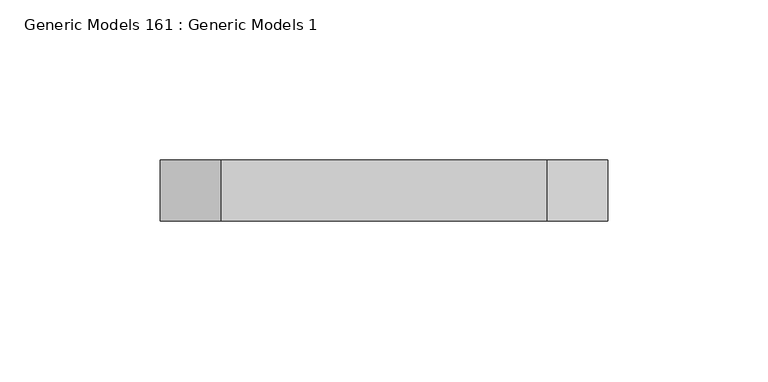
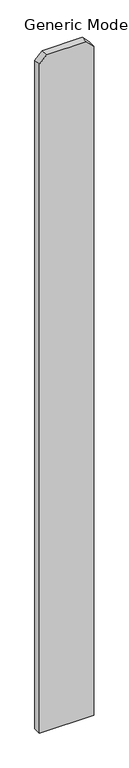
"""IFC4 building model written with IfcOpenShell, lengths in millimetres: proxy geometry, Generic Models 161 : Generic Models 1."""

from ifc_helpers import new_model, si_unit, frame, origin, place, context, project, spatial, polyline, outline, extrude, source, transform, mapped, element, save


def generic_models_161_generic_models_1_fa77210a(model_context):
    return source(origin(), model_context, "Body", "SweptSolid", [
        extrude(outline(polyline([(76.2, 54532.2125), (1885.95, 54532.2125), (1905.0, 54513.1625), (1905.0, 54411.5625), (1885.95, 54392.5125), (76.2, 54392.5125), (76.2, 54532.2125)])), frame((0.0, 547.6875, 0.0), z_axis=(0.0, 1.0, 0.0), x_axis=(0.0, 0.0, 1.0)), (0.0, 0.0, 1.0), 19.05),
    ])


if __name__ == "__main__":
    model = new_model("IFC4")
    model_context = context("Model", 3, world=origin())
    ifc_project = project(units=[si_unit("LENGTHUNIT", "METRE", prefix="MILLI")], contexts=[model_context])
    site = spatial("IfcSite", under=ifc_project)
    building = spatial("IfcBuilding", under=site)
    placement = place(None, origin())
    generic_models_161_generic_models_1_shape = generic_models_161_generic_models_1_fa77210a(model_context)
    element("IfcBuildingElementProxy", 1, Name="Generic Models 161 : Generic Models 1", ObjectType="Generic Models 161 : Generic Models 1", at=placement, inside=building, context=model_context, shape_type="MappedRepresentation", body=[
        mapped(generic_models_161_generic_models_1_shape, transform((0.0, 0.0, 0.0), x_axis=(1.0, 0.0, 0.0), y_axis=(0.0, 1.0, 0.0), z_axis=(0.0, 0.0, 1.0))),
    ])
    save(model, "model.ifc")

# Revit data of these elements
# Element 1 (IfcBuildingElementProxy, "Generic Models 161 : Generic Models 1")
#   Materials on its faces: "VERTICAL 1X6 CEDAR PLANKS W/ CLEAR WOOD SEALER"
# Materials
#   "VERTICAL 1X6 CEDAR PLANKS W/ CLEAR WOOD SEALER": class "Wood", colour RGB 234 198 147, transparency 0, Description = "Pinus Echinata", Cost = 0
